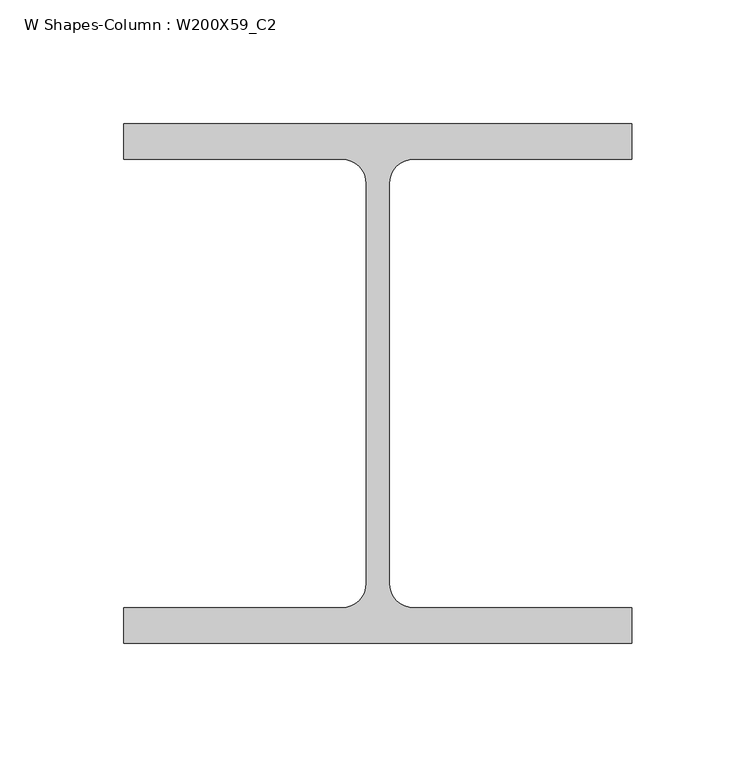
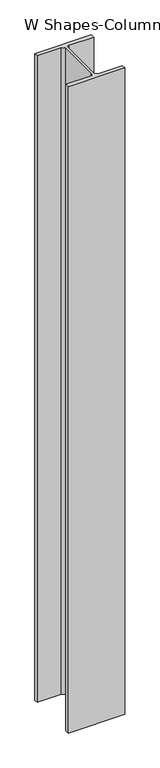
"""IFC4 building model written with IfcOpenShell, lengths in millimetres: column geometry, W Shapes-Column : W200X59_C2."""

import ifcopenshell
import ifcopenshell.guid

model = None  # the IFC model being written
_history = None  # IfcOwnerHistory: only IFC2X3 demands one
_inside = {}  # id of a spatial element -> (the spatial element, [elements in it])
_under = {}  # id of a project, library or spatial element -> (it, [spatial elements below it])
_declared = {}  # id of a project -> (the project, [libraries it declares])
_typed = {}  # id of a type object -> (the type object, [elements of that type])
_made_of = {}  # id of a material, layer set ... -> (it, [elements and type objects made of it])


def new_model(schema):
    """Start an empty IFC model of exactly this schema.

    Asked for "IFC4X3", IfcOpenShell would pick the latest addendum, in which some entities
    have other attributes; the version numbers below select the first issue.
    IFC2X3 requires an IfcOwnerHistory on every rooted entity: one is made here for all.
    """
    global model, _history
    if schema == "IFC4X3":
        model = ifcopenshell.file(schema_version=(4, 3, 0, 0))
    else:
        model = ifcopenshell.file(schema=schema)
    _inside.clear()
    _under.clear()
    _declared.clear()
    _typed.clear()
    _made_of.clear()
    _history = None
    if model.schema == "IFC2X3":
        org = make("IfcOrganization", Name="unknown")
        user = make(
            "IfcPersonAndOrganization",
            ThePerson=make("IfcPerson", FamilyName="unknown"),
            TheOrganization=org,
        )
        app = make(
            "IfcApplication",
            ApplicationDeveloper=org,
            Version="unknown",
            ApplicationFullName="unknown",
            ApplicationIdentifier="unknown",
        )
        _history = make(
            "IfcOwnerHistory",
            OwningUser=user,
            OwningApplication=app,
            ChangeAction="ADDED",
            CreationDate=0,
        )
    return model


def make(cls, **values):
    """One entity of the class cls with the attributes given. An attribute that is None is left unset."""
    return model.create_entity(
        cls, **{name: value for name, value in values.items() if value is not None}
    )


def rooted(cls, **values):
    """An entity with a GlobalId (a new one), such as an element, a storey or a relation."""
    return make(cls, GlobalId=ifcopenshell.guid.new(), OwnerHistory=_history, **values)


def si_unit(unit_type, name, prefix=None):
    """IfcSIUnit, for example si_unit("LENGTHUNIT", "METRE", prefix="MILLI")."""
    return make("IfcSIUnit", UnitType=unit_type, Prefix=prefix, Name=name)


def assignment(units):
    """IfcUnitAssignment: the units of a project."""
    return None if units is None else make("IfcUnitAssignment", Units=units)


def point(xyz):
    """IfcCartesianPoint."""
    return None if xyz is None else make("IfcCartesianPoint", Coordinates=xyz)


def direction(xyz):
    """IfcDirection."""
    return None if xyz is None else make("IfcDirection", DirectionRatios=xyz)


def frame(location, z_axis=None, x_axis=None):
    """IfcAxis2Placement3D, a coordinate frame: its origin and axes. An axis left out is left unset."""
    return make(
        "IfcAxis2Placement3D",
        Location=point(location),
        Axis=direction(z_axis),
        RefDirection=direction(x_axis),
    )


def frame_2d(location, x_axis=None):
    """IfcAxis2Placement2D, a coordinate frame in the plane: its origin and x axis."""
    return make(
        "IfcAxis2Placement2D", Location=point(location), RefDirection=direction(x_axis)
    )


def origin():
    """The frame at (0, 0, 0) with its axes left unset."""
    return frame((0.0, 0.0, 0.0))


def place(relative_to, where):
    """IfcLocalPlacement: puts the frame where relative to a parent placement (None: the world)."""
    return make(
        "IfcLocalPlacement", PlacementRelTo=relative_to, RelativePlacement=where
    )


def context(
    kind, dimensions, precision=None, world=None, true_north=None, identifier=None
):
    """IfcGeometricRepresentationContext, for example the 3D "Model" context."""
    return make(
        "IfcGeometricRepresentationContext",
        ContextIdentifier=identifier,
        ContextType=kind,
        CoordinateSpaceDimension=dimensions,
        Precision=precision,
        WorldCoordinateSystem=world,
        TrueNorth=true_north,
    )


def project(units=None, contexts=None):
    """IfcProject with its units and contexts."""
    return rooted(
        "IfcProject",
        Name="project",
        RepresentationContexts=contexts,
        UnitsInContext=assignment(units),
    )


def spatial(cls, under=None, at=None, **own):
    """A site, building, storey or space (cls), placed at a placement, below another one or the project."""
    s = rooted(cls, ObjectPlacement=at, **own)
    if under is not None:
        _under.setdefault(under.id(), (under, []))[1].append(s)
    return s


def polyline(points):
    """IfcPolyline through the points."""
    return make("IfcPolyline", Points=[point(p) for p in points])


def circle_curve(where, radius):
    """IfcCircle in the frame where."""
    return make("IfcCircle", Position=where, Radius=radius)


def trimmed(basis, trim1, trim2, sense, master):
    """IfcTrimmedCurve: the piece of a basis curve between two trims."""
    return make(
        "IfcTrimmedCurve",
        BasisCurve=basis,
        Trim1=trim1,
        Trim2=trim2,
        SenseAgreement=sense,
        MasterRepresentation=master,
    )


def segment(curve, same_sense, transition):
    """IfcCompositeCurveSegment."""
    return make(
        "IfcCompositeCurveSegment",
        Transition=transition,
        SameSense=same_sense,
        ParentCurve=curve,
    )


def composite_curve(segments, self_intersect=None):
    """IfcCompositeCurve: segments joined end to end."""
    return make("IfcCompositeCurve", Segments=segments, SelfIntersect=self_intersect)


def outline(outer, holes=None, kind="AREA"):
    """IfcArbitraryClosedProfileDef: a profile drawn as a closed curve; with holes, ...WithVoids."""
    if holes is None:
        return make("IfcArbitraryClosedProfileDef", ProfileType=kind, OuterCurve=outer)
    return make(
        "IfcArbitraryProfileDefWithVoids",
        ProfileType=kind,
        OuterCurve=outer,
        InnerCurves=holes,
    )


def extrude(swept, where, along, depth):
    """IfcExtrudedAreaSolid: the profile swept, set in the frame where, extruded along a direction by depth."""
    return make(
        "IfcExtrudedAreaSolid",
        SweptArea=swept,
        Position=where,
        ExtrudedDirection=direction(along),
        Depth=depth,
    )


def shape(context_of_items, identifier, shape_type, items):
    """IfcShapeRepresentation: the items that make up one representation, for example the "Body"."""
    return make(
        "IfcShapeRepresentation",
        ContextOfItems=context_of_items,
        RepresentationIdentifier=identifier,
        RepresentationType=shape_type,
        Items=items,
    )


def source(mapping_origin, context_of_items, identifier, shape_type, items):
    """IfcRepresentationMap: a shape defined once, which mapped items show again and again."""
    return make(
        "IfcRepresentationMap",
        MappingOrigin=mapping_origin,
        MappedRepresentation=shape(context_of_items, identifier, shape_type, items),
    )


def transform(
    local_origin,
    x_axis=None,
    y_axis=None,
    z_axis=None,
    scale=None,
    scale2=None,
    scale3=None,
    uniform=True,
):
    """IfcCartesianTransformationOperator3D, or its non-uniform kind. x_axis, y_axis, z_axis: its Axis1, 2, 3."""
    if uniform:
        return make(
            "IfcCartesianTransformationOperator3D",
            Axis1=direction(x_axis),
            Axis2=direction(y_axis),
            LocalOrigin=point(local_origin),
            Scale=scale,
            Axis3=direction(z_axis),
        )
    return make(
        "IfcCartesianTransformationOperator3DnonUniform",
        Axis1=direction(x_axis),
        Axis2=direction(y_axis),
        LocalOrigin=point(local_origin),
        Scale=scale,
        Axis3=direction(z_axis),
        Scale2=scale2,
        Scale3=scale3,
    )


def mapped(mapping_source, mapping_target):
    """IfcMappedItem: shows the shape of a source again, moved by a transform."""
    return make(
        "IfcMappedItem", MappingSource=mapping_source, MappingTarget=mapping_target
    )


def made_of(thing, what):
    """Note that an element or type object is made of a material, layer set ...; save() writes the relation."""
    if what is not None:
        _made_of.setdefault(what.id(), (what, []))[1].append(thing)
    return thing


def element(
    cls,
    number,
    at=None,
    inside=None,
    cuts=None,
    type_object=None,
    material=None,
    context=None,
    identifier="Body",
    shape_type=None,
    held_by="IfcProductDefinitionShape",
    body=None,
    shapes=None,
    **own,
):
    """One element of the class cls, such as IfcWall. Its Tag is "e" and its number.

    at: its placement. inside: the storey or other place that contains it. cuts: it is an
    opening in that element (IfcRelVoidsElement). A single representation is given by context,
    identifier, shape_type and body (its items); several are given by shapes. held_by: the class
    of the entity that holds the representations. save() writes the other relations.
    """
    e = rooted(cls, Tag="e%d" % number, ObjectPlacement=at, **own)
    if body is not None:
        shapes = [shape(context, identifier, shape_type, body)]
    if shapes is not None:
        e.Representation = make(held_by, Representations=shapes)
    if inside is not None:
        _inside.setdefault(inside.id(), (inside, []))[1].append(e)
    if cuts is not None:
        rooted(
            "IfcRelVoidsElement", RelatingBuildingElement=cuts, RelatedOpeningElement=e
        )
    if type_object is not None:
        _typed.setdefault(type_object.id(), (type_object, []))[1].append(e)
    return made_of(e, material)


def aggregate(whole, parts):
    """IfcRelAggregates: a whole, such as a stair, and the parts it consists of."""
    return rooted("IfcRelAggregates", RelatingObject=whole, RelatedObjects=parts)


def save(model, path):
    """Write the relations noted so far, then the file.

    IfcRelAggregates (storeys below a building ...), IfcRelContainedInSpatialStructure (elements
    in a storey), IfcRelDefinesByType, IfcRelAssociatesMaterial and IfcRelDeclares: one each for
    every whole, place, type object, material and project.
    """
    for whole, parts in _under.values():
        aggregate(whole, parts)
    for where, things in _inside.values():
        rooted(
            "IfcRelContainedInSpatialStructure",
            RelatedElements=things,
            RelatingStructure=where,
        )
    for kind, things in _typed.values():
        rooted("IfcRelDefinesByType", RelatedObjects=things, RelatingType=kind)
    for what, things in _made_of.values():
        rooted("IfcRelAssociatesMaterial", RelatedObjects=things, RelatingMaterial=what)
    for by, libraries in _declared.values():
        rooted("IfcRelDeclares", RelatingContext=by, RelatedDefinitions=libraries)
    model.write(path)


def w_shapes_column_w200x59_c2_42a61b42(model_context):
    return source(origin(), model_context, "Body", "SweptSolid", [
        extrude(outline(composite_curve([segment(polyline([(102.489, 104.775), (102.489, 90.551), (14.5796, 90.551)]), True, "CONTINUOUS"), segment(trimmed(circle_curve(frame_2d((14.5796, 80.5434)), 10.0076), [point((14.5796, 90.551))], [point((4.572, 80.5434))], True, "CARTESIAN"), True, "CONTINUOUS"), segment(polyline([(4.572, 80.5434), (4.572, -80.5434)]), True, "CONTINUOUS"), segment(trimmed(circle_curve(frame_2d((14.5796, -80.5434)), 10.0076), [point((4.572, -80.5434))], [point((14.5796, -90.551))], True, "CARTESIAN"), True, "CONTINUOUS"), segment(polyline([(14.5796, -90.551), (102.489, -90.551), (102.489, -104.775), (-102.489, -104.775), (-102.489, -90.551), (-14.5796, -90.551)]), True, "CONTINUOUS"), segment(trimmed(circle_curve(frame_2d((-14.5796, -80.5434)), 10.0076), [point((-14.5796, -90.551))], [point((-4.572, -80.5434))], True, "CARTESIAN"), True, "CONTINUOUS"), segment(polyline([(-4.572, -80.5434), (-4.572, 80.5434)]), True, "CONTINUOUS"), segment(trimmed(circle_curve(frame_2d((-14.5796, 80.5434)), 10.0076), [point((-4.572, 80.5434))], [point((-14.5796, 90.551))], True, "CARTESIAN"), True, "CONTINUOUS"), segment(polyline([(-14.5796, 90.551), (-102.489, 90.551), (-102.489, 104.775), (102.489, 104.775)]), True, "CONTINUOUS")], self_intersect=False)), frame((0.0, 0.0, 10066.0), z_axis=(0.0, 0.0, 1.0), x_axis=(1.0, 0.0, 0.0)), (0.0, 0.0, 1.0), 2484.0),
    ])


if __name__ == "__main__":
    model = new_model("IFC4")
    model_context = context("Model", 3, world=origin())
    ifc_project = project(units=[si_unit("LENGTHUNIT", "METRE", prefix="MILLI")], contexts=[model_context])
    site = spatial("IfcSite", under=ifc_project)
    building = spatial("IfcBuilding", under=site)
    placement = place(None, origin())
    w_shapes_column_w200x59_c2_shape = w_shapes_column_w200x59_c2_42a61b42(model_context)
    element("IfcColumn", 1, ObjectType="W Shapes-Column : W200X59_C2", at=placement, inside=building, context=model_context, shape_type="MappedRepresentation", body=[
        mapped(w_shapes_column_w200x59_c2_shape, transform((0.0, 0.0, 0.0), x_axis=(1.0, 0.0, 0.0), y_axis=(0.0, 1.0, 0.0), z_axis=(0.0, 0.0, 1.0))),
    ])
    save(model, "model.ifc")

# Revit data of these elements
# Type "W Shapes-Column : W200X59_C2"
#   Section Name Key = "W8x40"
#   Assembly Code = "B10"
#   Width = 20.4978 cm
#   Web Thickness = 0.9144 cm
#   Web Fillet = 1.0008 cm
#   Warping Constant = 194957.0 cm⁶
#   Torsional Moment of Inertia = 46.6179 cm⁴
#   Section Area = 75.4837 cm²
#   Plastic Modulus weak axis = 303.161 cm³
#   Plastic Modulus strong axis = 652.205 cm³
#   Perimeter = 1.20396 m²/m
#   Nominal Weight = 59.5266 kgf/m
#   Moment of Inertia weak axis = 2043.70 cm⁴
#   Moment of Inertia strong axis = 6076.98 cm⁴
#   Height = 20.955 cm
#   Flange Thickness = 1.4224 cm
#   Elastic Modulus weak axis = 199.922 cm³
#   Elastic Modulus strong axis = 581.741 cm³
#   Clear Web Height = 19.05 cm
#   Centroid Vertical = 10.4775 cm
#   Centroid Horizontal = 10.2489 cm
#   Bolt Spacing = 13.97 cm
#   Structural Material [instance default] = Steel ASTM A992
#   Principal Axes Angle = 0
# Element 1 (IfcColumn, "W Shapes-Column : W200X59_C2")
#   Structural Material = none
# Materials
#   "Steel ASTM A992": class "Metal", colour RGB 199 199 199, transparency 0, Description = "Structural steel 50ksi", Cost = 0
